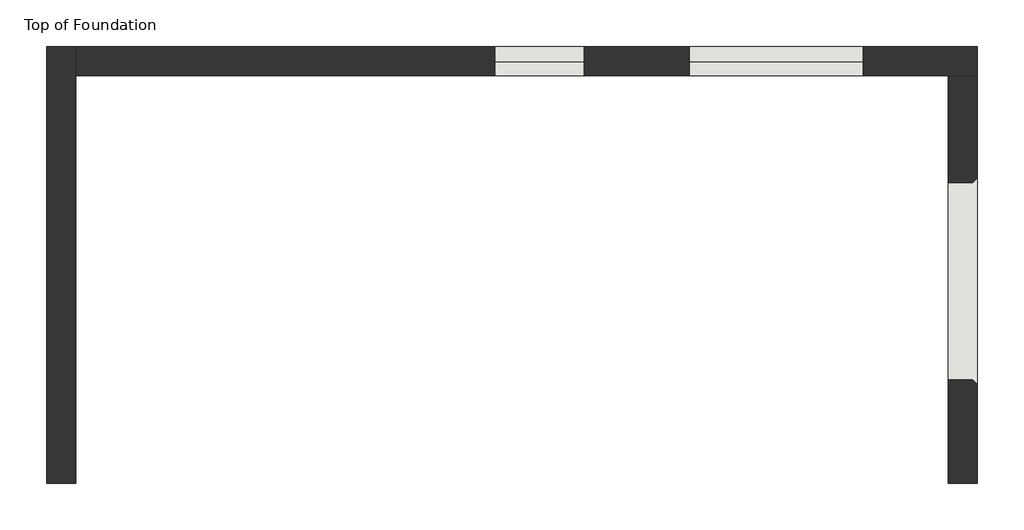
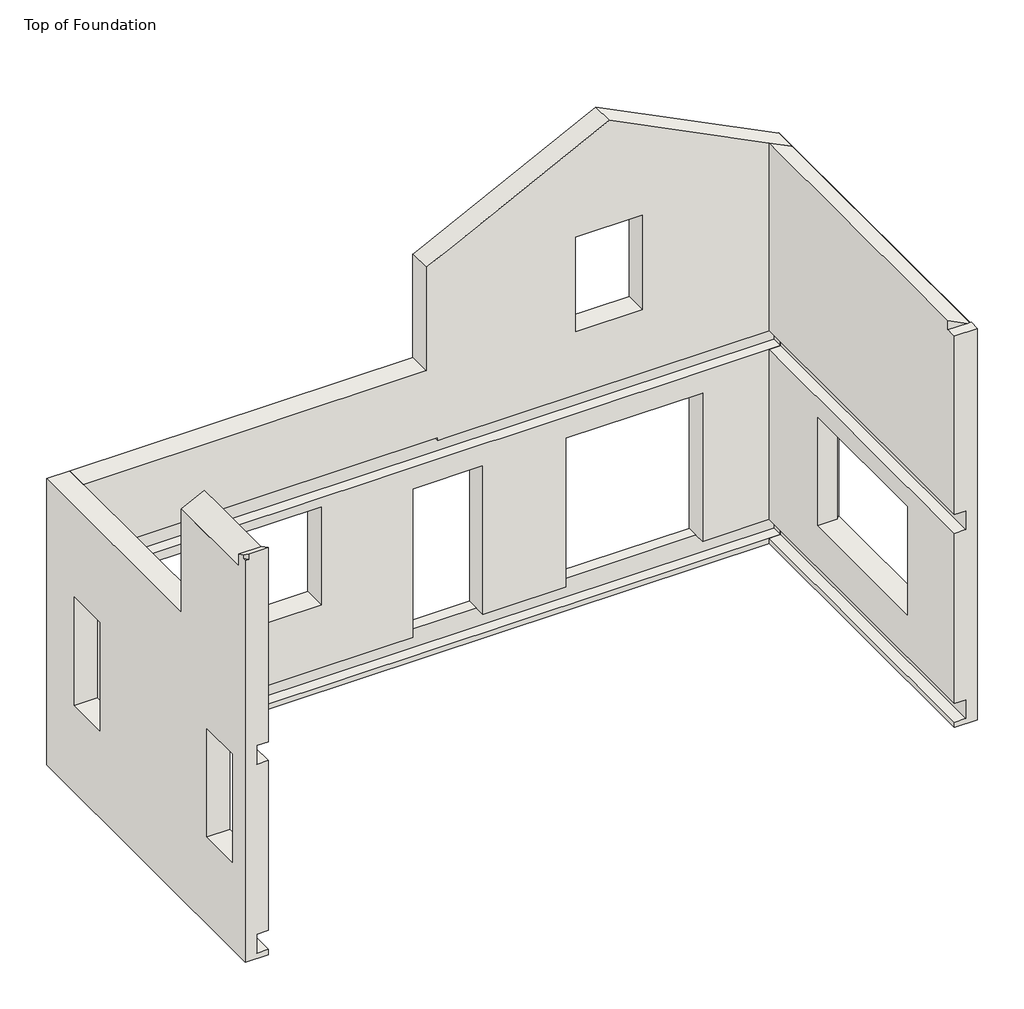
# One storey: 3 walls.
"""IFC4 building model written with IfcOpenShell, lengths in millimetres."""

from ifc_helpers import new_model, si_unit, origin, place, context, project, spatial, faceted_brep, element, save

model = new_model("IFC4")

# Units and contexts
model_context = context("Model", 3, world=origin())
ifc_project = project(units=[si_unit("LENGTHUNIT", "METRE", prefix="MILLI")], contexts=[model_context])

# Site, building, storey
site = spatial("IfcSite", under=ifc_project)
building = spatial("IfcBuilding", under=site)
storey = spatial("IfcBuildingStorey", under=building, Name="Top of Foundation", Elevation=-349.25)

# Walls
placement = place(None, origin())
element("IfcWall", 1, ObjectType="Exterior - Brick on Mtl. Stud", at=placement, inside=storey, context=model_context, shape_type="Brep", body=[
    faceted_brep([(-5671.6803068, 3152.0888758, -349.25), (-5671.6803068, 7558.9888758, -349.25), (-5671.6803068, 7876.4888758, -349.25), (-5671.6803068, 7876.4888758, 3810.0), (-5671.6803068, 7558.9888758, 3810.0), (-5671.6803068, 4676.0888758, 3810.0), (-5671.6803068, 4676.0888758, 5468.9375), (-5671.6803068, 4358.5888758, 5468.9375), (-5671.6803068, 3304.4888758, 5468.9375), (-5671.6803068, 3304.4888758, 5488.5342644), (-5671.6803068, 3152.0888758, 5564.7342644), (-5671.6803068, 3152.0888758, 2743.2), (-5671.6803068, 4358.5888758, 2743.2), (-5671.6803068, 4514.1638758, 2743.2), (-5671.6803068, 4514.1638758, 2781.3), (-5671.6803068, 4676.0888758, 2781.3), (-5671.6803068, 7558.9888758, 2781.3), (-5671.6803068, 7714.5638758, 2781.3), (-5671.6803068, 7714.5638758, 2470.15), (-5671.6803068, 7558.9888758, 2470.15), (-5671.6803068, 7219.2638758, 2470.15), (-5671.6803068, 7219.2638758, 914.4), (-5671.6803068, 6609.6638758, 914.4), (-5671.6803068, 6609.6638758, 2470.15), (-5671.6803068, 4066.4888758, 2470.15), (-5671.6803068, 4066.4888758, 914.4), (-5671.6803068, 3456.8888758, 914.4), (-5671.6803068, 3456.8888758, 2470.15), (-5671.6803068, 3152.0888758, 2470.15), (-5671.6803068, 3152.0888758, 0.0), (-5671.6803068, 7558.9888758, 0.0), (-5671.6803068, 7714.5638758, 0.0), (-5671.6803068, 7714.5638758, -273.05), (-5671.6803068, 7558.9888758, -273.05), (-5671.6803068, 3152.0888758, -273.05), (-5989.1803068, 7876.4888758, -349.25), (-5989.1803068, 3152.0888758, -349.25), (-5989.1803068, 3152.0888758, 5486.4), (-5989.1803068, 3199.7138758, 5486.4), (-5989.1803068, 3199.7138758, 5540.9217644), (-5989.1803068, 3304.4888758, 5488.5342644), (-5989.1803068, 3304.4888758, 5312.3217644), (-5989.1803068, 4676.0888758, 5312.3217644), (-5989.1803068, 4676.0888758, 3810.0), (-5989.1803068, 7876.4888758, 3810.0), (-5989.1803068, 3456.8888758, 2489.2), (-5989.1803068, 3456.8888758, 914.4), (-5989.1803068, 4066.4888758, 914.4), (-5989.1803068, 4066.4888758, 2489.2), (-5989.1803068, 6609.6638758, 2489.2), (-5989.1803068, 6609.6638758, 914.4), (-5989.1803068, 7219.2638758, 914.4), (-5989.1803068, 7219.2638758, 2489.2), (-5827.2553068, 3152.0888758, -273.05), (-5827.2553068, 3152.0888758, 0.0), (-5827.2553068, 3152.0888758, 2470.15), (-5827.2553068, 3152.0888758, 2743.2), (-5941.5553068, 3152.0888758, 5564.7342644), (-5941.5553068, 3152.0888758, 5486.4), (-5984.911778, 4676.0888758, 5312.3217644), (-5937.286778, 3304.4888758, 5336.1342644), (-5984.911778, 3304.4888758, 5312.3217644), (-5827.2553068, 3456.8888758, 2489.2), (-5827.2553068, 3456.8888758, 2470.15), (-5827.2553068, 4066.4888758, 2470.15), (-5827.2553068, 4066.4888758, 2489.2), (-5827.2553068, 6609.6638758, 2489.2), (-5827.2553068, 6609.6638758, 2470.15), (-5827.2553068, 7219.2638758, 2470.15), (-5827.2553068, 7219.2638758, 2489.2), (-5827.2553068, 7714.5638758, -273.05), (-5827.2553068, 7714.5638758, 0.0), (-5827.2553068, 7714.5638758, 2470.15), (-5827.2553068, 4514.1638758, 2470.15), (-5827.2553068, 4514.1638758, 2743.2), (-5827.2553068, 7714.5638758, 2781.3), (-5827.2553068, 4514.1638758, 2781.3)], [[[0, 1, 2, 3, 4, 5, 6, 7, 8, 9, 10, 11, 12, 13, 14, 15, 16, 17, 18, 19, 20, 21, 22, 23, 24, 25, 26, 27, 28, 29, 30, 31, 32, 33, 34]], [[35, 36, 37, 38, 39, 40, 41, 42, 43, 44], [45, 46, 47, 48], [49, 50, 51, 52]], [[2, 1, 0, 36, 35]], [[5, 4, 3, 44, 43]], [[37, 36, 0, 34, 53, 54, 29, 28, 55, 56, 11, 10, 57, 58]], [[3, 2, 35, 44]], [[6, 5, 43, 42, 59]], [[41, 40, 9, 8, 60, 61]], [[38, 37, 58]], [[38, 58, 57, 39]], [[8, 7, 6, 59, 61, 60]], [[42, 41, 61, 59]], [[10, 9, 40, 39, 57]], [[46, 45, 62, 63, 27, 26]], [[47, 46, 26, 25]], [[48, 47, 25, 24, 64, 65]], [[45, 48, 65, 62]], [[50, 49, 66, 67, 23, 22]], [[51, 50, 22, 21]], [[52, 51, 21, 20, 68, 69]], [[49, 52, 69, 66]], [[70, 53, 34, 33, 32]], [[71, 31, 30, 29, 54]], [[71, 70, 32, 31]], [[70, 71, 54, 53]], [[72, 68, 20, 19, 18]], [[64, 24, 23, 67, 73]], [[63, 55, 28, 27]], [[56, 74, 13, 12, 11]], [[55, 63, 62, 65, 64, 73, 67, 66, 69, 68, 72, 75, 76, 74, 56]], [[76, 75, 17, 16, 15, 14]], [[75, 72, 18, 17]], [[74, 76, 14, 13]]]),
])
element("IfcWall", 2, ObjectType="Exterior - Brick on Mtl. Stud", at=placement, inside=storey, context=model_context, shape_type="Brep", body=[
    faceted_brep([(-5671.6803068, 7558.9888758, -349.25), (3751.7196932, 7558.9888758, -349.25), (4069.2196932, 7558.9888758, -349.25), (4069.2196932, 7558.9888758, 5312.3217644), (4064.9511643, 7558.9888758, 5312.3217644), (3751.7196932, 7558.9888758, 5468.9375), (1554.6196932, 7558.9888758, 6567.4875), (-642.4803068, 7558.9888758, 5468.9375), (-955.711778, 7558.9888758, 5312.3217644), (-959.9803068, 7558.9888758, 5312.3217644), (-959.9803068, 7558.9888758, 3810.0), (-5671.6803068, 7558.9888758, 3810.0), (-5671.6803068, 7558.9888758, 2781.3), (-798.0553068, 7558.9888758, 2781.3), (-798.0553068, 7558.9888758, 2743.2), (-642.4803068, 7558.9888758, 2743.2), (3907.2946932, 7558.9888758, 2743.2), (3907.2946932, 7558.9888758, 2470.15), (43.3196932, 7558.9888758, 2470.15), (-77.3303068, 7558.9888758, 2470.15), (-1480.6803068, 7558.9888758, 2470.15), (-1601.3303068, 7558.9888758, 2470.15), (-5671.6803068, 7558.9888758, 2470.15), (-5671.6803068, 7558.9888758, 0.0), (-1601.3303068, 7558.9888758, 0.0), (-1480.6803068, 7558.9888758, 0.0), (-1144.1303068, 7558.9888758, 0.0), (-1144.1303068, 7558.9888758, 2159.0), (-178.9303068, 7558.9888758, 2159.0), (-178.9303068, 7558.9888758, 0.0), (-77.3303068, 7558.9888758, 0.0), (43.3196932, 7558.9888758, 0.0), (957.7196932, 7558.9888758, 0.0), (957.7196932, 7558.9888758, 2159.0), (2837.3196932, 7558.9888758, 2159.0), (2837.3196932, 7558.9888758, 0.0), (3907.2946932, 7558.9888758, 0.0), (3907.2946932, 7558.9888758, -273.05), (-5671.6803068, 7558.9888758, -273.05), (1097.4196932, 7558.9888758, 3657.6), (1097.4196932, 7558.9888758, 5029.2), (2011.8196932, 7558.9888758, 5029.2), (2011.8196932, 7558.9888758, 3657.6), (-2399.8428068, 7558.9888758, 2336.8), (-2399.8428068, 7558.9888758, 914.4), (-4838.2428068, 7558.9888758, 914.4), (-4838.2428068, 7558.9888758, 2336.8), (4069.2196932, 7876.4888758, -349.25), (-5671.6803068, 7876.4888758, -349.25), (-5671.6803068, 7876.4888758, 3810.0), (-959.9803068, 7876.4888758, 3810.0), (-959.9803068, 7876.4888758, 5312.3217644), (-955.711778, 7876.4888758, 5312.3217644), (1554.6196932, 7876.4888758, 6567.4875), (4064.9511643, 7876.4888758, 5312.3217644), (4069.2196932, 7876.4888758, 5312.3217644), (1097.4196932, 7876.4888758, 5029.2), (1097.4196932, 7876.4888758, 3657.6), (2011.8196932, 7876.4888758, 3657.6), (2011.8196932, 7876.4888758, 5029.2), (-1144.1303068, 7876.4888758, 2159.0), (-1144.1303068, 7876.4888758, 0.0), (-178.9303068, 7876.4888758, 0.0), (-178.9303068, 7876.4888758, 2159.0), (-2399.8428068, 7876.4888758, 914.4), (-2399.8428068, 7876.4888758, 2336.8), (-4838.2428068, 7876.4888758, 2336.8), (-4838.2428068, 7876.4888758, 914.4), (2837.3196932, 7876.4888758, 0.0), (2837.3196932, 7876.4888758, 2159.0), (957.7196932, 7876.4888758, 2159.0), (957.7196932, 7876.4888758, 0.0), (4069.2196932, 7571.6888758, -349.25), (-5671.6803068, 7714.5638758, -273.05), (-5671.6803068, 7714.5638758, 0.0), (-5671.6803068, 7714.5638758, 2470.15), (-5671.6803068, 7714.5638758, 2781.3), (-1144.1303068, 7714.5638758, 0.0), (-178.9303068, 7714.5638758, 0.0), (2837.3196932, 7714.5638758, 0.0), (957.7196932, 7714.5638758, 0.0), (3907.2946932, 7714.5638758, -273.05), (3907.2946932, 7714.5638758, 0.0), (3907.2946932, 7714.5638758, 2470.15), (-798.0553068, 7714.5638758, 2470.15), (-798.0553068, 7714.5638758, 2743.2), (3907.2946932, 7714.5638758, 2743.2), (-798.0553068, 7714.5638758, 2781.3)], [[[0, 1, 2, 3, 4, 5, 6, 7, 8, 9, 10, 11, 12, 13, 14, 15, 16, 17, 18, 19, 20, 21, 22, 23, 24, 25, 26, 27, 28, 29, 30, 31, 32, 33, 34, 35, 36, 37, 38], [39, 40, 41, 42], [43, 44, 45, 46]], [[47, 48, 49, 50, 51, 52, 53, 54, 55], [56, 57, 58, 59], [60, 61, 62, 63], [64, 65, 66, 67], [68, 69, 70, 71]], [[2, 1, 0, 48, 47, 72]], [[11, 10, 50, 49]], [[3, 2, 72, 47, 55]], [[11, 49, 48, 0, 38, 73, 74, 23, 22, 75, 76, 12]], [[10, 9, 51, 50]], [[51, 9, 8, 52]], [[8, 7, 6, 53, 52]], [[6, 5, 4, 54, 53]], [[3, 55, 54, 4]], [[57, 56, 40, 39]], [[58, 57, 39, 42]], [[59, 58, 42, 41]], [[56, 59, 41, 40]], [[27, 26, 77, 61, 60]], [[28, 27, 60, 63]], [[29, 28, 63, 62, 78]], [[62, 61, 77, 78]], [[44, 64, 67, 45]], [[65, 43, 46, 66]], [[64, 44, 43, 65]], [[66, 46, 45, 67]], [[69, 68, 79, 35, 34]], [[70, 69, 34, 33]], [[71, 70, 33, 32, 80]], [[68, 71, 80, 79]], [[37, 81, 73, 38]], [[79, 82, 36, 35]], [[78, 80, 32, 31, 30, 29]], [[74, 77, 26, 25, 24, 23]], [[81, 82, 79, 80, 78, 77, 74, 73]], [[82, 81, 37, 36]], [[75, 22, 21, 20, 19, 18, 17, 83, 84]], [[85, 86, 16, 15, 14]], [[75, 84, 83, 86, 85, 87, 76]], [[86, 83, 17, 16]], [[76, 87, 13, 12]], [[87, 85, 14, 13]]]),
])
element("IfcWall", 3, ObjectType="Exterior - Brick on Mtl. Stud", at=placement, inside=storey, context=model_context, shape_type="Brep", body=[
    faceted_brep([(3751.7196932, 7558.9888758, -349.25), (3751.7196932, 3152.0888758, -349.25), (3751.7196932, 3152.0888758, -273.05), (3751.7196932, 7558.9888758, -273.05), (3751.7196932, 3304.4888758, 5336.1342644), (3751.7196932, 3304.4888758, 5468.9375), (3751.7196932, 3844.2388758, 5468.9375), (3751.7196932, 3964.8888758, 5468.9375), (3751.7196932, 7558.9888758, 5468.9375), (3751.7196932, 7558.9888758, 2743.2), (3751.7196932, 3964.8888758, 2743.2), (3751.7196932, 3844.2388758, 2743.2), (3751.7196932, 3152.0888758, 2743.2), (3751.7196932, 3152.0888758, 5336.1342644), (3751.7196932, 7558.9888758, 0.0), (3751.7196932, 3152.0888758, 0.0), (3751.7196932, 3152.0888758, 2470.15), (3751.7196932, 7558.9888758, 2470.15), (3751.7196932, 6404.8763758, 2184.4), (3751.7196932, 4271.2763758, 2184.4), (3751.7196932, 4271.2763758, 609.6), (3751.7196932, 6404.8763758, 609.6), (4069.2196932, 3152.0888758, -349.25), (4069.2196932, 7558.9888758, -349.25), (4069.2196932, 7558.9888758, 5312.3217644), (4069.2196932, 3304.4888758, 5312.3217644), (4069.2196932, 3304.4888758, 5336.1342644), (4069.2196932, 3152.0888758, 5336.1342644), (4069.2196932, 4221.8849671, 2184.4), (4069.2196932, 6454.2677845, 2184.4), (4069.2196932, 6454.2677845, 609.6), (4069.2196932, 4221.8849671, 609.6), (3907.2946932, 3152.0888758, 2743.2), (3907.2946932, 3152.0888758, 2470.15), (3907.2946932, 3152.0888758, 0.0), (3907.2946932, 3152.0888758, -273.05), (3907.2946932, 7558.9888758, -273.05), (3907.2946932, 7558.9888758, 0.0), (3907.2946932, 7558.9888758, 2470.15), (3907.2946932, 7558.9888758, 2743.2), (4064.9511643, 7558.9888758, 5312.3217644), (4064.9511643, 3304.4888758, 5312.3217644), (4017.3261643, 3304.4888758, 5336.1342644), (4019.8282845, 6404.8763758, 2184.4), (4019.8282845, 4271.2763758, 2184.4), (4019.8282845, 6404.8763758, 609.6), (4019.8282845, 4271.2763758, 609.6)], [[[0, 1, 2, 3]], [[4, 5, 6, 7, 8, 9, 10, 11, 12, 13]], [[14, 15, 16, 17], [18, 19, 20, 21]], [[22, 23, 24, 25, 26, 27], [28, 29, 30, 31]], [[1, 0, 23, 22]], [[22, 27, 13, 12, 32, 33, 16, 15, 34, 35, 2, 1]], [[24, 23, 0, 3, 36, 37, 14, 17, 38, 39, 9, 8, 40]], [[26, 25, 41, 42]], [[4, 13, 27, 26, 42]], [[8, 7, 6, 5, 42, 41, 40]], [[25, 24, 40, 41]], [[5, 4, 42]], [[43, 29, 28, 44, 19, 18]], [[45, 21, 20, 46, 31, 30]], [[43, 18, 21, 45]], [[19, 44, 46, 20]], [[44, 28, 31, 46]], [[29, 43, 45, 30]], [[35, 36, 3, 2]], [[37, 34, 15, 14]], [[36, 35, 34, 37]], [[33, 38, 17, 16]], [[39, 32, 12, 11, 10, 9]], [[38, 33, 32, 39]]]),
])

save(model, "model.ifc")

# Revit data of these elements
# Type "Exterior - Brick on Mtl. Stud"
#   Assembly Code = "B2010158"
#   Layers, outside or top first: 0' - 3 5/8" "Brick, Common" (function 4); 0' - 2" "Air" (function 3); 0' - 0" "Air Infiltration Barrier" (function 100); 0' - 0 3/4" "Plywood, Sheathing" (function 2); 0' - 5 1/2" "Metal Stud Layer" (function 1); 0' - 0" "Vapor Retarder" (function 100); 0' - 0 5/8" "Gypsum Wall Board" (function 5)
# Elements 1, 2 (IfcWall, "Exterior - Brick on Mtl. Stud")
#   Top Offset = 0' - 0"
#   Base Offset = 0' - 0"
#   wall height = 19' - 1 3/4"
#   Phase Created = New Construction
#   Base Constraint = Top of Foundation
#   Top Constraint = Roof
#   Materials on its faces: "Default Wall", "Brick, Common", "Gypsum Wall Board"
# Element 3 (IfcWall, "Exterior - Brick on Mtl. Stud")
#   Top Offset = 0' - 0"
#   Base Offset = 0' - 0"
#   wall height = 19' - 1 3/4"
#   Phase Created = New Construction
#   Base Constraint = Top of Foundation
#   Top Constraint = Roof
#   Materials on its faces: "Default Wall", "Gypsum Wall Board", "Brick, Common"
# Materials
#   "Brick, Common": class "Masonry", colour RGB 170 98 104, transparency 0, Description = "Common brick", Cost = 0
#   "Air": class "Gas", colour RGB 255 255 255, transparency 0, Description = "Air", Cost = 0
#   "Air Infiltration Barrier": class "Generic", colour RGB 127 127 127, transparency 0, Description = "physical material", Cost = 0
#   "Plywood, Sheathing": class "Wood", colour RGB 193 140 64, transparency 0, Description = "Plywood, sheathing grade", Cost = 0
#   "Metal Stud Layer": class "Metal", colour RGB 199 199 199, transparency 0, Description = "Light gauge steel framing, thermal air layer", Cost = 0
#   "Vapor Retarder": class "Generic", colour RGB 127 127 127, transparency 0, Description = "Polyethylene film membrane", Cost = 0
#   "Gypsum Wall Board": class "Generic", colour RGB 127 127 127, transparency 0, Description = "Gypsum Wall Board", Cost = 0
#   "Default Wall": class "Miscellaneous", colour RGB 128 128 128, transparency 0, Cost = 0
